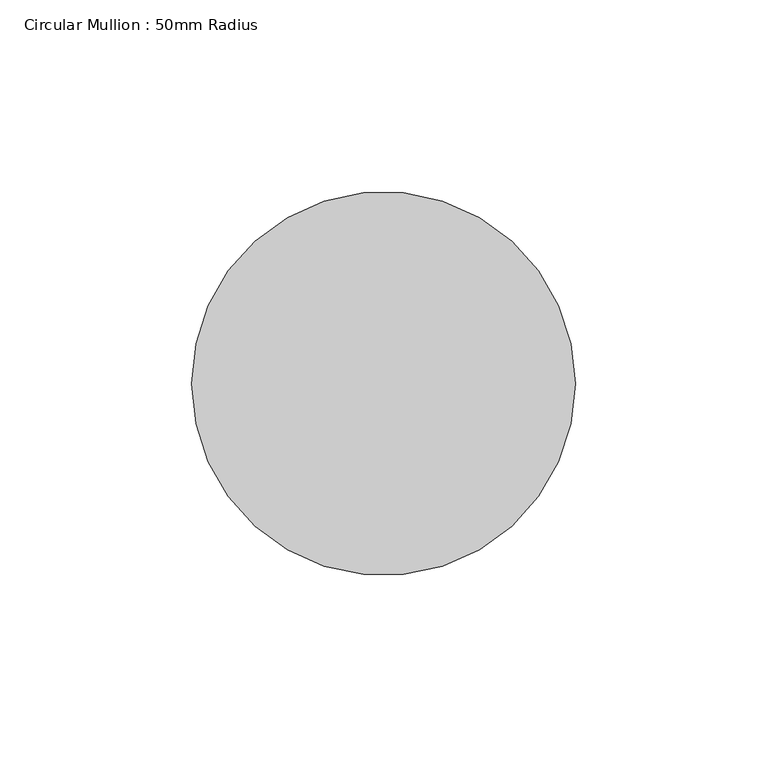
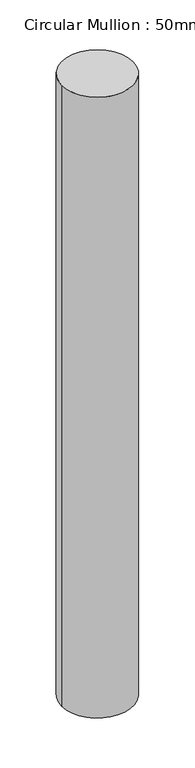
"""IFC4 building model written with IfcOpenShell, lengths in millimetres: member geometry, Circular Mullion : 50mm Radius."""

from ifc_helpers import new_model, si_unit, point, frame, origin, origin_2d, place, context, project, spatial, circle_curve, trimmed, segment, composite_curve, outline, extrude, source, transform, mapped, element, save


def circular_mullion_50mm_radius_d7d47897(model_context):
    return source(origin(), model_context, "Body", "SweptSolid", [
        extrude(outline(composite_curve([segment(trimmed(circle_curve(origin_2d(), 50.0), [point((50.0, 0.0))], [point((-50.0, 0.0))], False, "CARTESIAN"), True, "CONTINUOUS"), segment(trimmed(circle_curve(origin_2d(), 50.0), [point((-50.0, 0.0))], [point((50.0, 0.0))], False, "CARTESIAN"), True, "CONTINUOUS")], self_intersect=False)), frame((0.0, 0.0, -918.3803059), z_axis=(0.0, 0.0, 1.0), x_axis=(1.0, 0.0, 0.0)), (0.0, 0.0, 1.0), 918.3803059),
    ])


if __name__ == "__main__":
    model = new_model("IFC4")
    model_context = context("Model", 3, world=origin())
    ifc_project = project(units=[si_unit("LENGTHUNIT", "METRE", prefix="MILLI")], contexts=[model_context])
    site = spatial("IfcSite", under=ifc_project)
    building = spatial("IfcBuilding", under=site)
    placement = place(None, origin())
    circular_mullion_50mm_radius_shape = circular_mullion_50mm_radius_d7d47897(model_context)
    element("IfcMember", 1, ObjectType="Circular Mullion : 50mm Radius", at=placement, inside=building, context=model_context, shape_type="MappedRepresentation", body=[
        mapped(circular_mullion_50mm_radius_shape, transform((0.0, 0.0, 0.0), x_axis=(1.0, 0.0, 0.0), y_axis=(0.0, 1.0, 0.0), z_axis=(0.0, 0.0, 1.0))),
    ])
    save(model, "model.ifc")

# Revit data of these elements
# Type "Circular Mullion : 50mm Radius"
#   built-in parameter 1007350 = 0.164042 (stored number, unit not read)
# Element 1 (IfcMember, "Circular Mullion : 50mm Radius")
#   Materials on its faces: "Aluminium"
# Materials
#   "Aluminium": class "Metal", colour RGB 247 247 247, transparency 0, Description = "Aluminium 6061", Cost = 0
